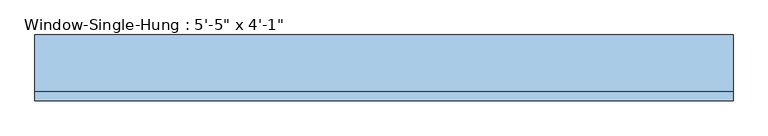
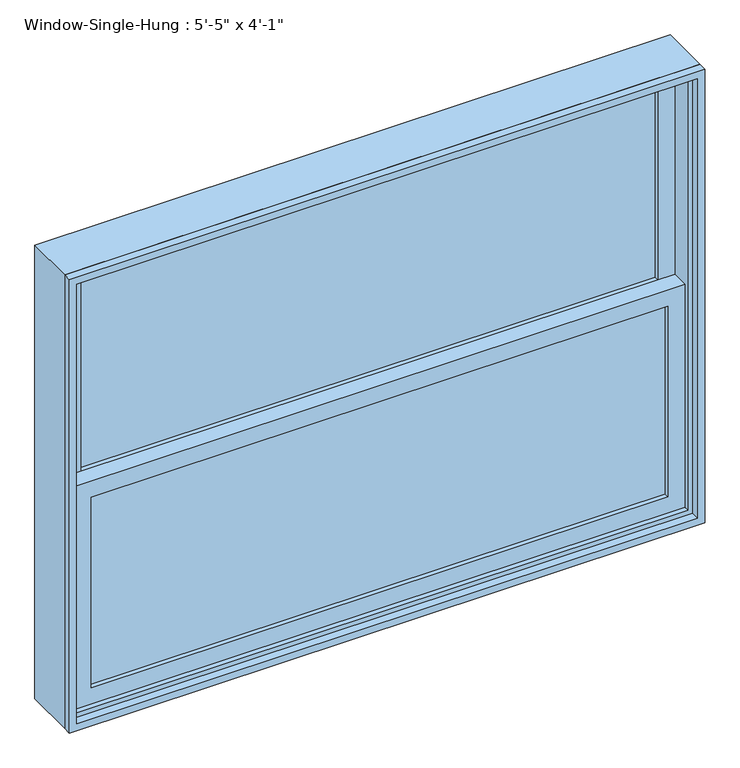
"""IFC4 building model written with IfcOpenShell, lengths in millimetres: window geometry."""

from ifc_helpers import new_model, si_unit, frame, origin, place, context, project, spatial, polyline, outline, extrude, source, transform, mapped, element, save


def window_bdfed6d5(model_context):
    return source(origin(), model_context, "Body", "SweptSolid", [
        extrude(outline(polyline([(749.3, -1.5875), (749.3, -7.9375), (-749.3, -7.9375), (-749.3, -1.5875), (749.3, -1.5875)])), frame((0.0, 0.0, 990.6), z_axis=(0.0, 0.0, 1.0), x_axis=(1.0, 0.0, 0.0)), (0.0, 0.0, 1.0), 523.875),
        extrude(outline(polyline([(-749.3, -14.2875), (749.3, -14.2875), (749.3, -20.6375), (-749.3, -20.6375), (-749.3, -14.2875)])), frame((0.0, 0.0, 990.6), z_axis=(0.0, 0.0, 1.0), x_axis=(1.0, 0.0, 0.0)), (0.0, 0.0, 1.0), 523.875),
        extrude(outline(polyline([(749.3, 42.8625), (749.3, 36.5125), (-749.3, 36.5125), (-749.3, 42.8625), (749.3, 42.8625)])), frame((0.0, 0.0, 1558.925), z_axis=(0.0, 0.0, 1.0), x_axis=(1.0, 0.0, 0.0)), (0.0, 0.0, 1.0), 523.875),
        extrude(outline(polyline([(-749.3, 30.1625), (749.3, 30.1625), (749.3, 23.8125), (-749.3, 23.8125), (-749.3, 30.1625)])), frame((0.0, 0.0, 1558.925), z_axis=(0.0, 0.0, 1.0), x_axis=(1.0, 0.0, 0.0)), (0.0, 0.0, 1.0), 523.875),
        extrude(outline(polyline([(1558.925, -793.75), (946.15, -793.75), (946.15, 793.75), (1558.925, 793.75), (1558.925, -793.75)]), holes=[polyline([(1514.475, 749.3), (990.6, 749.3), (990.6, -749.3), (1514.475, -749.3), (1514.475, 749.3)])]), frame((0.0, -33.3375, 0.0), z_axis=(0.0, 1.0, 0.0), x_axis=(0.0, 0.0, 1.0)), (0.0, 0.0, 1.0), 44.45),
        extrude(outline(polyline([(2127.25, -793.75), (1514.475, -793.75), (1514.475, 793.75), (2127.25, 793.75), (2127.25, -793.75)]), holes=[polyline([(2082.8, 749.3), (1558.925, 749.3), (1558.925, -749.3), (2082.8, -749.3), (2082.8, 749.3)])]), frame((0.0, 11.1125, 0.0), z_axis=(0.0, 1.0, 0.0), x_axis=(0.0, 0.0, 1.0)), (0.0, 0.0, 1.0), 44.45),
        extrude(outline(polyline([(2159.0, -825.5), (914.4, -825.5), (914.4, 825.5), (2159.0, 825.5), (2159.0, -825.5)]), holes=[polyline([(2127.25, 793.75), (946.15, 793.75), (946.15, -793.75), (2127.25, -793.75), (2127.25, 793.75)])]), frame((0.0, -46.0375, 0.0), z_axis=(0.0, 1.0, 0.0), x_axis=(0.0, 0.0, 1.0)), (0.0, 0.0, 1.0), 133.35),
        extrude(outline(polyline([(2159.0, 825.5), (2159.0, -825.5), (914.4, -825.5), (914.4, 825.5), (2159.0, 825.5)]), holes=[polyline([(2139.95, 806.45), (933.45, 806.45), (933.45, -806.45), (2139.95, -806.45), (2139.95, 806.45)])]), frame((0.0, -68.2625, 0.0), z_axis=(0.0, 1.0, 0.0), x_axis=(0.0, 0.0, 1.0)), (0.0, 0.0, 1.0), 22.225),
    ])


if __name__ == "__main__":
    model = new_model("IFC4")
    model_context = context("Model", 3, world=origin())
    ifc_project = project(units=[si_unit("LENGTHUNIT", "METRE", prefix="MILLI")], contexts=[model_context])
    site = spatial("IfcSite", under=ifc_project)
    building = spatial("IfcBuilding", under=site)
    placement = place(None, origin())
    window_shape = window_bdfed6d5(model_context)
    element("IfcWindow", 1, ObjectType="Window-Single-Hung : 5'-5\" x 4'-1\"", at=placement, inside=building, context=model_context, shape_type="MappedRepresentation", body=[
        mapped(window_shape, transform((0.0, 0.0, 0.0), x_axis=(1.0, 0.0, 0.0), y_axis=(0.0, 1.0, 0.0), z_axis=(0.0, 0.0, 1.0))),
    ])
    save(model, "model.ifc")

# Revit data of these elements
# Type "Window-Single-Hung : 5'-5\" x 4'-1\""
#   Type Mark = "27"
#   Fire Rating = "0.5h"
#   Construction Type Id = "DG-DR"
#   Assembly Code = "B2020100"
#   Analytic Construction = "Double glazing - domestic"
#   Wall Thickness [instance default] = 0' - 6"
#   Window Inset [instance default] = 0' - 0"
#   Visual Light Transmittance = 0.81
#   Thermal Resistance (R) = 0.319569 (m²·K)/W
#   Solar Heat Gain Coefficient = 0.76
#   Muntin Width = 4' - 11"
#   Muntin Height = 1' - 8 5/8"
#   Interior Wall Closure [instance default] = 0' - 1 1/2"
#   Rough Width = 5' - 5 1/2"
#   Rough Height = 4' - 1 1/2"
#   Frame Extension [instance default] = 0' - 1 1/4"
#   Exterior Wall Closure [instance default] = 0' - 0 1/2"
#   Extension Jamb [instance default] = 0' - 1 1/2"
#   Heat Transfer Coefficient (U) = 3.12929 W/(m²·K)
#   Height = 4' - 1"
#   Width = 5' - 5"
#   Top Muntin Visibility = yes
#   Indicator Visibility [instance default] = yes
#   Extension Jamb Visibility [instance default] = yes
#   Interior Trim Visibility [instance default] = yes
#   Exterior Trim Visibility [instance default] = yes
#   Bottom Muntin Visibility = yes
#   Muntin Pattern = Muntin Pattern_2x2 : Muntin Pattern_2x2
#   Interior Trim Material = Wood - Stained
#   Interior Trim = Trim-Window-Interior-Flat : Picture Frame
#   Exterior Trim Material = Clad - White
#   Exterior Trim = Trim-Window-Exterior-Flat : with Sill
#   Glass Panel Material = Glass
#   Exterior Frame Material = Clad - White
#   Interior Frame Material = Wood - Stained
#   Wall Closure = (empty or 0)
# Element 1 (IfcWindow, "Window-Single-Hung : 5'-5\" x 4'-1\"")
#   Wall Thickness = 0' - 5 3/8"
#   Extension Jamb = 0' - 0 7/8"
#   Materials on its faces: "Wood - Stained", "Glass", "Clad - White"
# Materials
#   "Wood - Stained": class "Wood", colour RGB 224 178 126, transparency 0, Cost = 0
#   "Clad - White": class "Wood", colour RGB 242 242 238, transparency 0, Cost = 0
#   "Glass": class "Glass", colour RGB 0 128 192, transparency 0.75, Description = "Soda Lime Glass", Cost = 0
